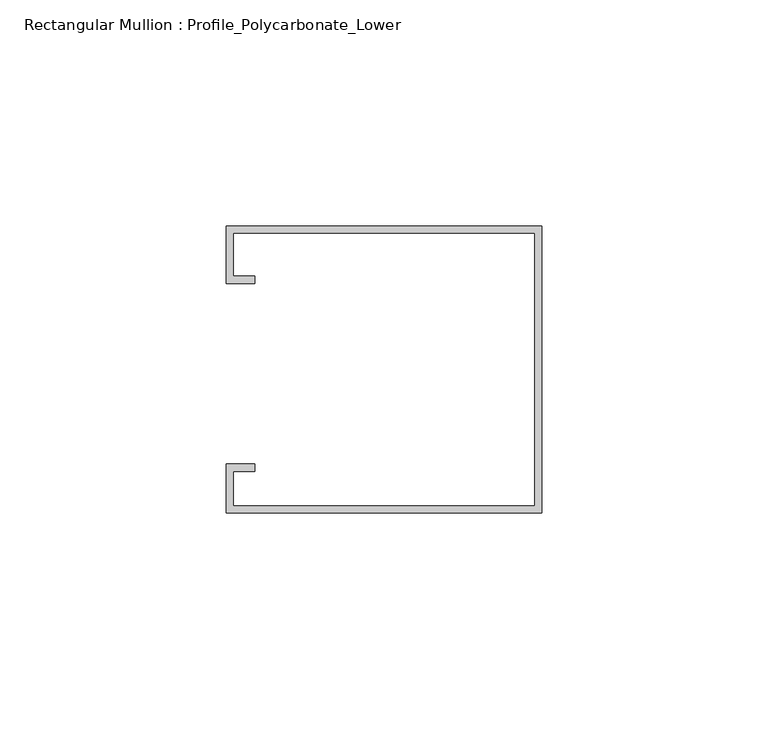
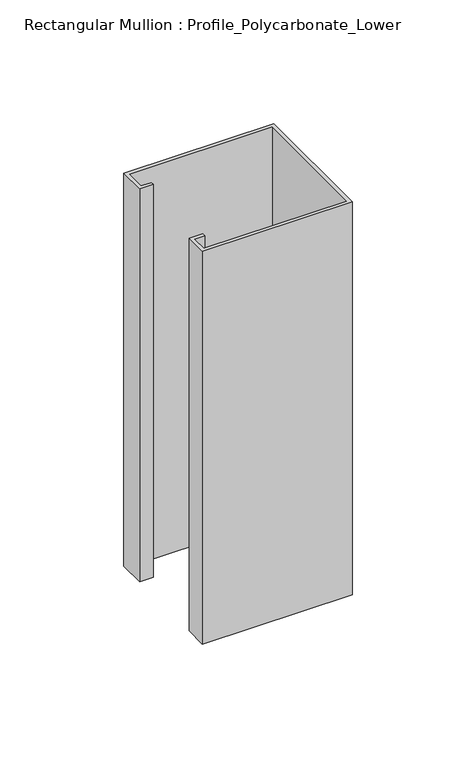
"""IFC4 building model written with IfcOpenShell, lengths in millimetres: member geometry, Rectangular Mullion : Profile_Polycarbonate_Lower."""

from ifc_helpers import new_model, si_unit, frame, origin, place, context, project, spatial, polyline, outline, extrude, source, transform, mapped, element, save


def rectangular_mullion_profile_polycarbonate_lower_5ca23ea1(model_context):
    return source(origin(), model_context, "Body", "SweptSolid", [
        extrude(outline(polyline([(0.0, 32.7), (0.0, -30.8), (-69.85, -30.8), (-69.85, -20.0), (-63.5, -20.0), (-63.5, -21.5875), (-68.2625, -21.5875), (-68.2625, -29.2125), (-1.5875, -29.2125), (-1.5875, 31.1125), (-68.2625, 31.1125), (-68.2625, 21.5875), (-63.5, 21.5875), (-63.5, 20.0), (-69.85, 20.0), (-69.85, 32.7), (0.0, 32.7)])), frame((0.0, 0.0, -193.675), z_axis=(0.0, 0.0, 1.0), x_axis=(1.0, 0.0, 0.0)), (0.0, 0.0, 1.0), 193.675),
    ])


if __name__ == "__main__":
    model = new_model("IFC4")
    model_context = context("Model", 3, world=origin())
    ifc_project = project(units=[si_unit("LENGTHUNIT", "METRE", prefix="MILLI")], contexts=[model_context])
    site = spatial("IfcSite", under=ifc_project)
    building = spatial("IfcBuilding", under=site)
    placement = place(None, origin())
    rectangular_mullion_profile_polycarbonate_lower_shape = rectangular_mullion_profile_polycarbonate_lower_5ca23ea1(model_context)
    element("IfcMember", 1, ObjectType="Rectangular Mullion : Profile_Polycarbonate_Lower", at=placement, inside=building, context=model_context, shape_type="MappedRepresentation", body=[
        mapped(rectangular_mullion_profile_polycarbonate_lower_shape, transform((0.0, 0.0, 0.0), x_axis=(1.0, 0.0, 0.0), y_axis=(0.0, 1.0, 0.0), z_axis=(0.0, 0.0, 1.0))),
    ])
    save(model, "model.ifc")

# Revit data of these elements
# Type "Rectangular Mullion : Profile_Polycarbonate_Lower"
#   built-in parameter 1007322 = 0.208333 (stored number, unit not read)
#   built-in parameter 1007321 = 0 (stored number, unit not read)
#   built-in parameter 1007320 = 0.00520833 (stored number, unit not read)
# Element 1 (IfcMember, "Rectangular Mullion : Profile_Polycarbonate_Lower")
#   Materials on its faces: "GALVANIZED UNISTRUT P5500, 1 5/8\" X 2 7/16\" OR ALUM. CHANNEL"
# Materials
#   "GALVANIZED UNISTRUT P5500, 1 5/8\" X 2 7/16\" OR ALUM. CHANNEL": class "Metal", colour RGB 244 244 244, transparency 0, Description = "Aluminum 6061", Cost = 0
